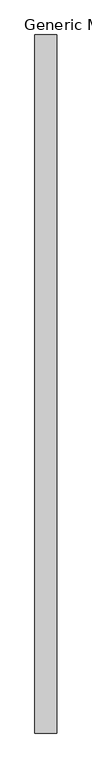
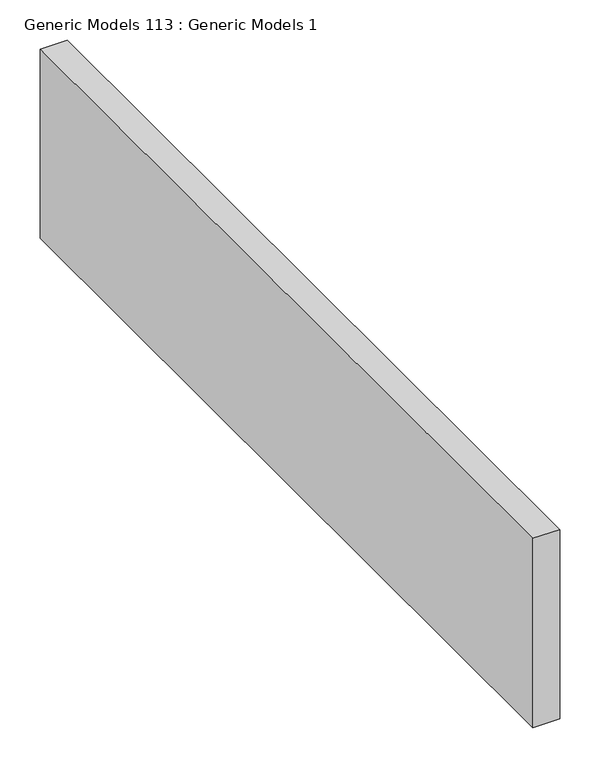
"""IFC4 building model written with IfcOpenShell, lengths in millimetres: proxy geometry, Generic Models 113 : Generic Models 1."""

from ifc_helpers import new_model, si_unit, frame, origin, place, context, project, spatial, polyline, outline, extrude, source, transform, mapped, element, save


def generic_models_113_generic_models_1_101608ab(model_context):
    return source(origin(), model_context, "Body", "SweptSolid", [
        extrude(outline(polyline([(52171.6, 0.0), (52133.5, 0.0), (52133.5, 1219.2), (52171.6, 1219.2), (52171.6, 0.0)])), frame((0.0, 0.0, 5222.478125), z_axis=(0.0, 0.0, 1.0), x_axis=(1.0, 0.0, 0.0)), (0.0, 0.0, 1.0), 285.75),
    ])


if __name__ == "__main__":
    model = new_model("IFC4")
    model_context = context("Model", 3, world=origin())
    ifc_project = project(units=[si_unit("LENGTHUNIT", "METRE", prefix="MILLI")], contexts=[model_context])
    site = spatial("IfcSite", under=ifc_project)
    building = spatial("IfcBuilding", under=site)
    placement = place(None, origin())
    generic_models_113_generic_models_1_shape = generic_models_113_generic_models_1_101608ab(model_context)
    element("IfcBuildingElementProxy", 1, Name="Generic Models 113 : Generic Models 1", ObjectType="Generic Models 113 : Generic Models 1", at=placement, inside=building, context=model_context, shape_type="MappedRepresentation", body=[
        mapped(generic_models_113_generic_models_1_shape, transform((0.0, 0.0, 0.0), x_axis=(1.0, 0.0, 0.0), y_axis=(0.0, 1.0, 0.0), z_axis=(0.0, 0.0, 1.0))),
    ])
    save(model, "model.ifc")

# Revit data of these elements
# Element 1 (IfcBuildingElementProxy, "Generic Models 113 : Generic Models 1")
#   Materials on its faces: "RIM BOARD - SIZE TO MATCH JOIST DEPTH"
# Materials
#   "RIM BOARD - SIZE TO MATCH JOIST DEPTH": class "Wood", colour RGB 234 198 147, transparency 0, Description = "Pinus Echinata", Cost = 0
